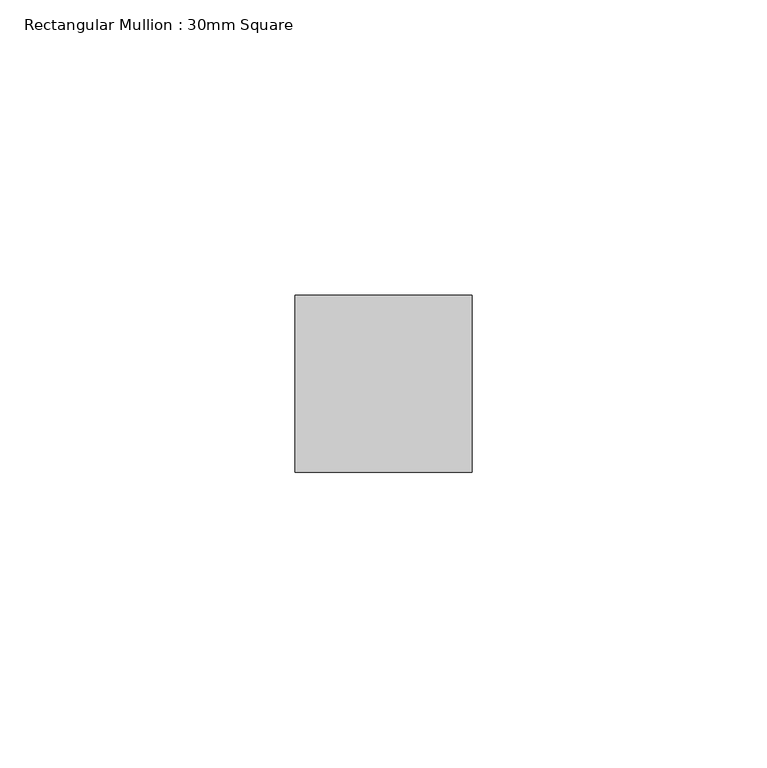
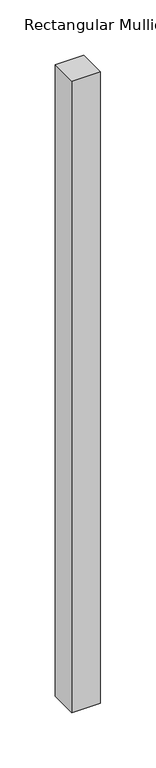
"""IFC4 building model written with IfcOpenShell, lengths in millimetres: member geometry, Rectangular Mullion : 30mm Square."""

from ifc_helpers import new_model, si_unit, frame, origin, place, context, project, spatial, polyline, outline, extrude, source, transform, mapped, element, save


def rectangular_mullion_30mm_square_db8d2200(model_context):
    return source(origin(), model_context, "Body", "SweptSolid", [
        extrude(outline(polyline([(15.0, 15.0), (15.0, -15.0), (-15.0, -15.0), (-15.0, 15.0), (15.0, 15.0)])), frame((0.0, 0.0, -698.3926374), z_axis=(0.0, 0.0, 1.0), x_axis=(1.0, 0.0, 0.0)), (0.0, 0.0, 1.0), 698.3926374),
    ])


if __name__ == "__main__":
    model = new_model("IFC4")
    model_context = context("Model", 3, world=origin())
    ifc_project = project(units=[si_unit("LENGTHUNIT", "METRE", prefix="MILLI")], contexts=[model_context])
    site = spatial("IfcSite", under=ifc_project)
    building = spatial("IfcBuilding", under=site)
    placement = place(None, origin())
    rectangular_mullion_30mm_square_shape = rectangular_mullion_30mm_square_db8d2200(model_context)
    element("IfcMember", 1, ObjectType="Rectangular Mullion : 30mm Square", at=placement, inside=building, context=model_context, shape_type="MappedRepresentation", body=[
        mapped(rectangular_mullion_30mm_square_shape, transform((0.0, 0.0, 0.0), x_axis=(1.0, 0.0, 0.0), y_axis=(0.0, 1.0, 0.0), z_axis=(0.0, 0.0, 1.0))),
    ])
    save(model, "model.ifc")

# Revit data of these elements
# Type "Rectangular Mullion : 30mm Square"
#   built-in parameter 1007304 = 0.0984252 (stored number, unit not read)
#   built-in parameter 1007301 = 0.0492126 (stored number, unit not read)
#   built-in parameter 1007300 = 0.0492126 (stored number, unit not read)
# Element 1 (IfcMember, "Rectangular Mullion : 30mm Square")
#   Materials on its faces: "Aluminum"
# Materials
#   "Aluminum": class "Metal", colour RGB 244 244 244, transparency 0, Description = "Aluminum 6061", Cost = 0
